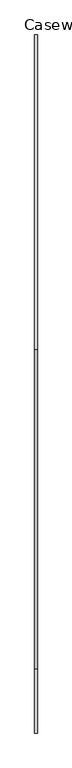
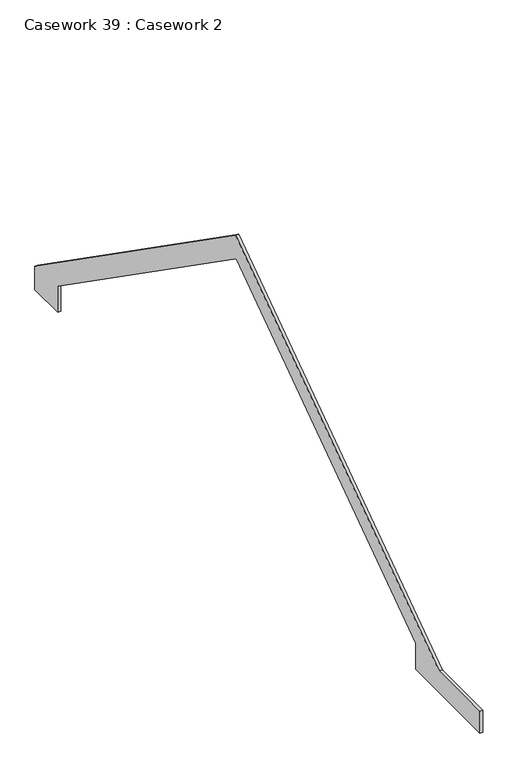
"""IFC4 building model written with IfcOpenShell, lengths in millimetres: furniture geometry, Casework 39 : Casework 2."""

import ifcopenshell
import ifcopenshell.guid

model = None  # the IFC model being written
_history = None  # IfcOwnerHistory: only IFC2X3 demands one
_inside = {}  # id of a spatial element -> (the spatial element, [elements in it])
_under = {}  # id of a project, library or spatial element -> (it, [spatial elements below it])
_declared = {}  # id of a project -> (the project, [libraries it declares])
_typed = {}  # id of a type object -> (the type object, [elements of that type])
_made_of = {}  # id of a material, layer set ... -> (it, [elements and type objects made of it])


def new_model(schema):
    """Start an empty IFC model of exactly this schema.

    Asked for "IFC4X3", IfcOpenShell would pick the latest addendum, in which some entities
    have other attributes; the version numbers below select the first issue.
    IFC2X3 requires an IfcOwnerHistory on every rooted entity: one is made here for all.
    """
    global model, _history
    if schema == "IFC4X3":
        model = ifcopenshell.file(schema_version=(4, 3, 0, 0))
    else:
        model = ifcopenshell.file(schema=schema)
    _inside.clear()
    _under.clear()
    _declared.clear()
    _typed.clear()
    _made_of.clear()
    _history = None
    if model.schema == "IFC2X3":
        org = make("IfcOrganization", Name="unknown")
        user = make(
            "IfcPersonAndOrganization",
            ThePerson=make("IfcPerson", FamilyName="unknown"),
            TheOrganization=org,
        )
        app = make(
            "IfcApplication",
            ApplicationDeveloper=org,
            Version="unknown",
            ApplicationFullName="unknown",
            ApplicationIdentifier="unknown",
        )
        _history = make(
            "IfcOwnerHistory",
            OwningUser=user,
            OwningApplication=app,
            ChangeAction="ADDED",
            CreationDate=0,
        )
    return model


def make(cls, **values):
    """One entity of the class cls with the attributes given. An attribute that is None is left unset."""
    return model.create_entity(
        cls, **{name: value for name, value in values.items() if value is not None}
    )


def rooted(cls, **values):
    """An entity with a GlobalId (a new one), such as an element, a storey or a relation."""
    return make(cls, GlobalId=ifcopenshell.guid.new(), OwnerHistory=_history, **values)


def si_unit(unit_type, name, prefix=None):
    """IfcSIUnit, for example si_unit("LENGTHUNIT", "METRE", prefix="MILLI")."""
    return make("IfcSIUnit", UnitType=unit_type, Prefix=prefix, Name=name)


def assignment(units):
    """IfcUnitAssignment: the units of a project."""
    return None if units is None else make("IfcUnitAssignment", Units=units)


def point(xyz):
    """IfcCartesianPoint."""
    return None if xyz is None else make("IfcCartesianPoint", Coordinates=xyz)


def direction(xyz):
    """IfcDirection."""
    return None if xyz is None else make("IfcDirection", DirectionRatios=xyz)


def frame(location, z_axis=None, x_axis=None):
    """IfcAxis2Placement3D, a coordinate frame: its origin and axes. An axis left out is left unset."""
    return make(
        "IfcAxis2Placement3D",
        Location=point(location),
        Axis=direction(z_axis),
        RefDirection=direction(x_axis),
    )


def origin():
    """The frame at (0, 0, 0) with its axes left unset."""
    return frame((0.0, 0.0, 0.0))


def place(relative_to, where):
    """IfcLocalPlacement: puts the frame where relative to a parent placement (None: the world)."""
    return make(
        "IfcLocalPlacement", PlacementRelTo=relative_to, RelativePlacement=where
    )


def context(
    kind, dimensions, precision=None, world=None, true_north=None, identifier=None
):
    """IfcGeometricRepresentationContext, for example the 3D "Model" context."""
    return make(
        "IfcGeometricRepresentationContext",
        ContextIdentifier=identifier,
        ContextType=kind,
        CoordinateSpaceDimension=dimensions,
        Precision=precision,
        WorldCoordinateSystem=world,
        TrueNorth=true_north,
    )


def project(units=None, contexts=None):
    """IfcProject with its units and contexts."""
    return rooted(
        "IfcProject",
        Name="project",
        RepresentationContexts=contexts,
        UnitsInContext=assignment(units),
    )


def spatial(cls, under=None, at=None, **own):
    """A site, building, storey or space (cls), placed at a placement, below another one or the project."""
    s = rooted(cls, ObjectPlacement=at, **own)
    if under is not None:
        _under.setdefault(under.id(), (under, []))[1].append(s)
    return s


def polyline(points):
    """IfcPolyline through the points."""
    return make("IfcPolyline", Points=[point(p) for p in points])


def outline(outer, holes=None, kind="AREA"):
    """IfcArbitraryClosedProfileDef: a profile drawn as a closed curve; with holes, ...WithVoids."""
    if holes is None:
        return make("IfcArbitraryClosedProfileDef", ProfileType=kind, OuterCurve=outer)
    return make(
        "IfcArbitraryProfileDefWithVoids",
        ProfileType=kind,
        OuterCurve=outer,
        InnerCurves=holes,
    )


def extrude(swept, where, along, depth):
    """IfcExtrudedAreaSolid: the profile swept, set in the frame where, extruded along a direction by depth."""
    return make(
        "IfcExtrudedAreaSolid",
        SweptArea=swept,
        Position=where,
        ExtrudedDirection=direction(along),
        Depth=depth,
    )


def shape(context_of_items, identifier, shape_type, items):
    """IfcShapeRepresentation: the items that make up one representation, for example the "Body"."""
    return make(
        "IfcShapeRepresentation",
        ContextOfItems=context_of_items,
        RepresentationIdentifier=identifier,
        RepresentationType=shape_type,
        Items=items,
    )


def source(mapping_origin, context_of_items, identifier, shape_type, items):
    """IfcRepresentationMap: a shape defined once, which mapped items show again and again."""
    return make(
        "IfcRepresentationMap",
        MappingOrigin=mapping_origin,
        MappedRepresentation=shape(context_of_items, identifier, shape_type, items),
    )


def transform(
    local_origin,
    x_axis=None,
    y_axis=None,
    z_axis=None,
    scale=None,
    scale2=None,
    scale3=None,
    uniform=True,
):
    """IfcCartesianTransformationOperator3D, or its non-uniform kind. x_axis, y_axis, z_axis: its Axis1, 2, 3."""
    if uniform:
        return make(
            "IfcCartesianTransformationOperator3D",
            Axis1=direction(x_axis),
            Axis2=direction(y_axis),
            LocalOrigin=point(local_origin),
            Scale=scale,
            Axis3=direction(z_axis),
        )
    return make(
        "IfcCartesianTransformationOperator3DnonUniform",
        Axis1=direction(x_axis),
        Axis2=direction(y_axis),
        LocalOrigin=point(local_origin),
        Scale=scale,
        Axis3=direction(z_axis),
        Scale2=scale2,
        Scale3=scale3,
    )


def mapped(mapping_source, mapping_target):
    """IfcMappedItem: shows the shape of a source again, moved by a transform."""
    return make(
        "IfcMappedItem", MappingSource=mapping_source, MappingTarget=mapping_target
    )


def made_of(thing, what):
    """Note that an element or type object is made of a material, layer set ...; save() writes the relation."""
    if what is not None:
        _made_of.setdefault(what.id(), (what, []))[1].append(thing)
    return thing


def element(
    cls,
    number,
    at=None,
    inside=None,
    cuts=None,
    type_object=None,
    material=None,
    context=None,
    identifier="Body",
    shape_type=None,
    held_by="IfcProductDefinitionShape",
    body=None,
    shapes=None,
    **own,
):
    """One element of the class cls, such as IfcWall. Its Tag is "e" and its number.

    at: its placement. inside: the storey or other place that contains it. cuts: it is an
    opening in that element (IfcRelVoidsElement). A single representation is given by context,
    identifier, shape_type and body (its items); several are given by shapes. held_by: the class
    of the entity that holds the representations. save() writes the other relations.
    """
    e = rooted(cls, Tag="e%d" % number, ObjectPlacement=at, **own)
    if body is not None:
        shapes = [shape(context, identifier, shape_type, body)]
    if shapes is not None:
        e.Representation = make(held_by, Representations=shapes)
    if inside is not None:
        _inside.setdefault(inside.id(), (inside, []))[1].append(e)
    if cuts is not None:
        rooted(
            "IfcRelVoidsElement", RelatingBuildingElement=cuts, RelatedOpeningElement=e
        )
    if type_object is not None:
        _typed.setdefault(type_object.id(), (type_object, []))[1].append(e)
    return made_of(e, material)


def aggregate(whole, parts):
    """IfcRelAggregates: a whole, such as a stair, and the parts it consists of."""
    return rooted("IfcRelAggregates", RelatingObject=whole, RelatedObjects=parts)


def save(model, path):
    """Write the relations noted so far, then the file.

    IfcRelAggregates (storeys below a building ...), IfcRelContainedInSpatialStructure (elements
    in a storey), IfcRelDefinesByType, IfcRelAssociatesMaterial and IfcRelDeclares: one each for
    every whole, place, type object, material and project.
    """
    for whole, parts in _under.values():
        aggregate(whole, parts)
    for where, things in _inside.values():
        rooted(
            "IfcRelContainedInSpatialStructure",
            RelatedElements=things,
            RelatingStructure=where,
        )
    for kind, things in _typed.values():
        rooted("IfcRelDefinesByType", RelatedObjects=things, RelatingType=kind)
    for what, things in _made_of.values():
        rooted("IfcRelAssociatesMaterial", RelatedObjects=things, RelatingMaterial=what)
    for by, libraries in _declared.values():
        rooted("IfcRelDeclares", RelatingContext=by, RelatedDefinitions=libraries)
    model.write(path)


def casework_39_casework_2_646cf92f(model_context):
    return source(origin(), model_context, "Body", "SweptSolid", [
        extrude(outline(polyline([(3156.9704867, 7937.1283557), (7125.8166964, 5158.1123216), (7125.8166964, 4875.3461918), (6675.8166964, 4875.3461918), (6675.8166964, 5190.0895255), (3151.1408768, 7658.0941041), (-400.040882, 5171.5298671), (-400.040882, 4860.0), (-1669.6462381, 4860.0), (-1669.6462381, 5121.8983063), (-863.5946969, 5121.8983063), (3156.9704867, 7937.1283557)])), frame((713.8336886, 0.0, 0.0), z_axis=(1.0, 0.0, 0.0), x_axis=(0.0, 1.0, 0.0)), (0.0, 0.0, 1.0), 33.2089356),
    ])


if __name__ == "__main__":
    model = new_model("IFC4")
    model_context = context("Model", 3, world=origin())
    ifc_project = project(units=[si_unit("LENGTHUNIT", "METRE", prefix="MILLI")], contexts=[model_context])
    site = spatial("IfcSite", under=ifc_project)
    building = spatial("IfcBuilding", under=site)
    placement = place(None, origin())
    casework_39_casework_2_shape = casework_39_casework_2_646cf92f(model_context)
    element("IfcFurniture", 1, ObjectType="Casework 39 : Casework 2", at=placement, inside=building, context=model_context, shape_type="MappedRepresentation", body=[
        mapped(casework_39_casework_2_shape, transform((0.0, 0.0, 0.0), x_axis=(1.0, 0.0, 0.0), y_axis=(0.0, 1.0, 0.0), z_axis=(0.0, 0.0, 1.0))),
    ])
    save(model, "model.ifc")

# Revit data of these elements
# Element 1 (IfcFurniture, "Casework 39 : Casework 2")
#   Materials on its faces: "Timber, Painted, White"
# Materials
#   "Timber, Painted, White": class "Wood", colour RGB 255 255 255, transparency 0, Comments = "Rendering appearance not upgraded ", Description = "Timber Barge Board, White Paint Finish", Cost = 0
